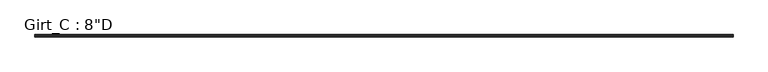
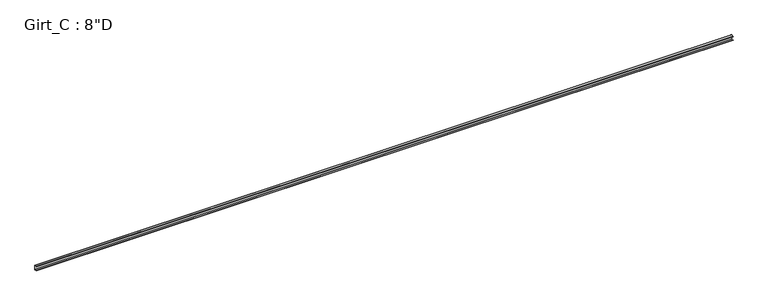
"""IFC4 building model written with IfcOpenShell, lengths in millimetres: beam geometry."""

from ifc_helpers import new_model, si_unit, point, frame, frame_2d, origin, place, context, project, spatial, polyline, circle_curve, trimmed, segment, composite_curve, outline, extrude, source, transform, mapped, element, save


def beam_fb6f6511(model_context):
    return source(origin(), model_context, "Body", "SweptSolid", [
        extrude(outline(composite_curve([segment(polyline([(-87.5109375, 101.6), (-3.3734375, 101.6)]), True, "CONTINUOUS"), segment(trimmed(circle_curve(frame_2d((-3.3734375, 96.8375)), 4.7625), [point((-3.3734375, 101.6))], [point((1.3890625, 96.8375))], False, "CARTESIAN"), True, "CONTINUOUS"), segment(polyline([(1.3890625, 96.8375), (1.3890625, -96.8375)]), True, "CONTINUOUS"), segment(trimmed(circle_curve(frame_2d((-3.3734375, -96.8375)), 4.7625), [point((1.3890625, -96.8375))], [point((-3.3734375, -101.6))], False, "CARTESIAN"), True, "CONTINUOUS"), segment(polyline([(-3.3734375, -101.6), (-87.5109375, -101.6), (-99.7792647, -86.979177), (-97.6510975, -85.1934327), (-86.2154765, -98.821875), (-3.2694106, -98.821875)]), True, "CONTINUOUS"), segment(trimmed(circle_curve(frame_2d((-3.3748024, -96.8389339)), 1.9857399), [point((-3.2694106, -98.821875))], [point((-1.3890625, -96.8389339))], True, "CARTESIAN"), True, "CONTINUOUS"), segment(polyline([(-1.3890625, -96.8389339), (-1.3890625, 96.8381931)]), True, "CONTINUOUS"), segment(trimmed(circle_curve(frame_2d((-3.3741066, 96.8381931)), 1.9850441), [point((-1.3890625, 96.8381931))], [point((-3.3005807, 98.821875))], True, "CARTESIAN"), True, "CONTINUOUS"), segment(polyline([(-3.3005807, 98.821875), (-86.2154765, 98.821875), (-97.6278742, 85.221109), (-99.7560415, 87.0068534), (-87.5109375, 101.6)]), True, "CONTINUOUS")], self_intersect=False)), frame((-15570.2, 0.0, 0.0), z_axis=(1.0, 0.0, 0.0), x_axis=(0.0, 1.0, 0.0)), (0.0, 0.0, 1.0), 31140.4),
    ])


if __name__ == "__main__":
    model = new_model("IFC4")
    model_context = context("Model", 3, world=origin())
    ifc_project = project(units=[si_unit("LENGTHUNIT", "METRE", prefix="MILLI")], contexts=[model_context])
    site = spatial("IfcSite", under=ifc_project)
    building = spatial("IfcBuilding", under=site)
    placement = place(None, origin())
    beam_shape = beam_fb6f6511(model_context)
    element("IfcBeam", 1, ObjectType="Girt_C : 8\"D", at=placement, inside=building, context=model_context, shape_type="MappedRepresentation", body=[
        mapped(beam_shape, transform((0.0, 0.0, 0.0), x_axis=(1.0, 0.0, 0.0), y_axis=(0.0, 1.0, 0.0), z_axis=(0.0, 0.0, 1.0))),
    ])
    save(model, "model.ifc")

# Revit data of these elements
# Type "Girt_C : 8\"D"
#   half leg = 0' - 1 3/4"
#   Web_Thickness = 0' - 0 7/64"
#   Length [instance default] = 10' - 0"
#   Leg_1 = 0' - 3 1/2"
#   Height = 0' - 8"
#   Structural Material [instance default] = none
# Element 1 (IfcBeam, "Girt_C : 8\"D")
#   Structural Material = CEE' SECTION (8.0x3.5C - SEE STRUCT. DWGS)
#   Materials on its faces: "CEE' SECTION (8.0x3.5C - SEE STRUCT. DWGS)"
# Materials
#   "CEE' SECTION (8.0x3.5C - SEE STRUCT. DWGS)": class "Metal", colour RGB 137 146 153, transparency 0, Description = "Steel, mill finish", Cost = 0
